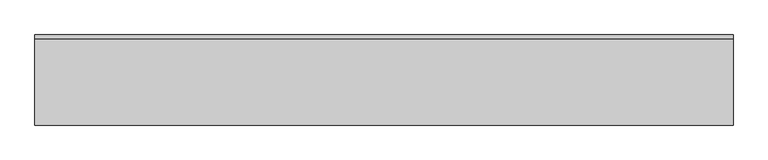
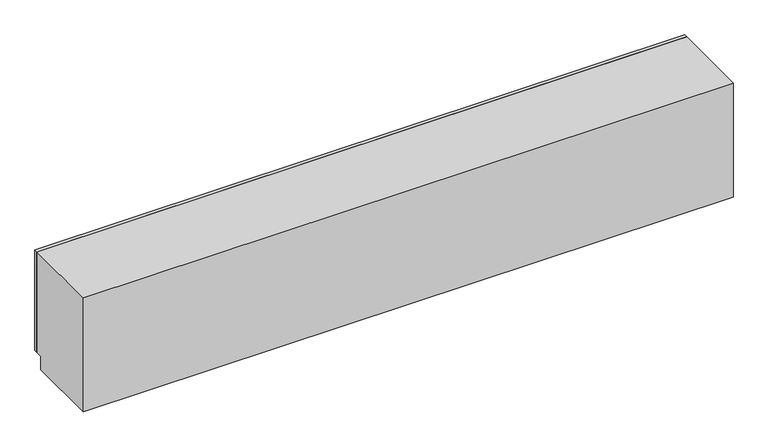
"""IFC4 building model written with IfcOpenShell, lengths in millimetres: furniture geometry, OD_CW_Base Cabinet : OD_CW_Base Cabinet."""

import ifcopenshell
import ifcopenshell.guid

model = None  # the IFC model being written
_history = None  # IfcOwnerHistory: only IFC2X3 demands one
_inside = {}  # id of a spatial element -> (the spatial element, [elements in it])
_under = {}  # id of a project, library or spatial element -> (it, [spatial elements below it])
_declared = {}  # id of a project -> (the project, [libraries it declares])
_typed = {}  # id of a type object -> (the type object, [elements of that type])
_made_of = {}  # id of a material, layer set ... -> (it, [elements and type objects made of it])


def new_model(schema):
    """Start an empty IFC model of exactly this schema.

    Asked for "IFC4X3", IfcOpenShell would pick the latest addendum, in which some entities
    have other attributes; the version numbers below select the first issue.
    IFC2X3 requires an IfcOwnerHistory on every rooted entity: one is made here for all.
    """
    global model, _history
    if schema == "IFC4X3":
        model = ifcopenshell.file(schema_version=(4, 3, 0, 0))
    else:
        model = ifcopenshell.file(schema=schema)
    _inside.clear()
    _under.clear()
    _declared.clear()
    _typed.clear()
    _made_of.clear()
    _history = None
    if model.schema == "IFC2X3":
        org = make("IfcOrganization", Name="unknown")
        user = make(
            "IfcPersonAndOrganization",
            ThePerson=make("IfcPerson", FamilyName="unknown"),
            TheOrganization=org,
        )
        app = make(
            "IfcApplication",
            ApplicationDeveloper=org,
            Version="unknown",
            ApplicationFullName="unknown",
            ApplicationIdentifier="unknown",
        )
        _history = make(
            "IfcOwnerHistory",
            OwningUser=user,
            OwningApplication=app,
            ChangeAction="ADDED",
            CreationDate=0,
        )
    return model


def make(cls, **values):
    """One entity of the class cls with the attributes given. An attribute that is None is left unset."""
    return model.create_entity(
        cls, **{name: value for name, value in values.items() if value is not None}
    )


def rooted(cls, **values):
    """An entity with a GlobalId (a new one), such as an element, a storey or a relation."""
    return make(cls, GlobalId=ifcopenshell.guid.new(), OwnerHistory=_history, **values)


def si_unit(unit_type, name, prefix=None):
    """IfcSIUnit, for example si_unit("LENGTHUNIT", "METRE", prefix="MILLI")."""
    return make("IfcSIUnit", UnitType=unit_type, Prefix=prefix, Name=name)


def assignment(units):
    """IfcUnitAssignment: the units of a project."""
    return None if units is None else make("IfcUnitAssignment", Units=units)


def point(xyz):
    """IfcCartesianPoint."""
    return None if xyz is None else make("IfcCartesianPoint", Coordinates=xyz)


def direction(xyz):
    """IfcDirection."""
    return None if xyz is None else make("IfcDirection", DirectionRatios=xyz)


def frame(location, z_axis=None, x_axis=None):
    """IfcAxis2Placement3D, a coordinate frame: its origin and axes. An axis left out is left unset."""
    return make(
        "IfcAxis2Placement3D",
        Location=point(location),
        Axis=direction(z_axis),
        RefDirection=direction(x_axis),
    )


def origin():
    """The frame at (0, 0, 0) with its axes left unset."""
    return frame((0.0, 0.0, 0.0))


def place(relative_to, where):
    """IfcLocalPlacement: puts the frame where relative to a parent placement (None: the world)."""
    return make(
        "IfcLocalPlacement", PlacementRelTo=relative_to, RelativePlacement=where
    )


def context(
    kind, dimensions, precision=None, world=None, true_north=None, identifier=None
):
    """IfcGeometricRepresentationContext, for example the 3D "Model" context."""
    return make(
        "IfcGeometricRepresentationContext",
        ContextIdentifier=identifier,
        ContextType=kind,
        CoordinateSpaceDimension=dimensions,
        Precision=precision,
        WorldCoordinateSystem=world,
        TrueNorth=true_north,
    )


def project(units=None, contexts=None):
    """IfcProject with its units and contexts."""
    return rooted(
        "IfcProject",
        Name="project",
        RepresentationContexts=contexts,
        UnitsInContext=assignment(units),
    )


def spatial(cls, under=None, at=None, **own):
    """A site, building, storey or space (cls), placed at a placement, below another one or the project."""
    s = rooted(cls, ObjectPlacement=at, **own)
    if under is not None:
        _under.setdefault(under.id(), (under, []))[1].append(s)
    return s


def polyline(points):
    """IfcPolyline through the points."""
    return make("IfcPolyline", Points=[point(p) for p in points])


def outline(outer, holes=None, kind="AREA"):
    """IfcArbitraryClosedProfileDef: a profile drawn as a closed curve; with holes, ...WithVoids."""
    if holes is None:
        return make("IfcArbitraryClosedProfileDef", ProfileType=kind, OuterCurve=outer)
    return make(
        "IfcArbitraryProfileDefWithVoids",
        ProfileType=kind,
        OuterCurve=outer,
        InnerCurves=holes,
    )


def extrude(swept, where, along, depth):
    """IfcExtrudedAreaSolid: the profile swept, set in the frame where, extruded along a direction by depth."""
    return make(
        "IfcExtrudedAreaSolid",
        SweptArea=swept,
        Position=where,
        ExtrudedDirection=direction(along),
        Depth=depth,
    )


def shape(context_of_items, identifier, shape_type, items):
    """IfcShapeRepresentation: the items that make up one representation, for example the "Body"."""
    return make(
        "IfcShapeRepresentation",
        ContextOfItems=context_of_items,
        RepresentationIdentifier=identifier,
        RepresentationType=shape_type,
        Items=items,
    )


def source(mapping_origin, context_of_items, identifier, shape_type, items):
    """IfcRepresentationMap: a shape defined once, which mapped items show again and again."""
    return make(
        "IfcRepresentationMap",
        MappingOrigin=mapping_origin,
        MappedRepresentation=shape(context_of_items, identifier, shape_type, items),
    )


def transform(
    local_origin,
    x_axis=None,
    y_axis=None,
    z_axis=None,
    scale=None,
    scale2=None,
    scale3=None,
    uniform=True,
):
    """IfcCartesianTransformationOperator3D, or its non-uniform kind. x_axis, y_axis, z_axis: its Axis1, 2, 3."""
    if uniform:
        return make(
            "IfcCartesianTransformationOperator3D",
            Axis1=direction(x_axis),
            Axis2=direction(y_axis),
            LocalOrigin=point(local_origin),
            Scale=scale,
            Axis3=direction(z_axis),
        )
    return make(
        "IfcCartesianTransformationOperator3DnonUniform",
        Axis1=direction(x_axis),
        Axis2=direction(y_axis),
        LocalOrigin=point(local_origin),
        Scale=scale,
        Axis3=direction(z_axis),
        Scale2=scale2,
        Scale3=scale3,
    )


def mapped(mapping_source, mapping_target):
    """IfcMappedItem: shows the shape of a source again, moved by a transform."""
    return make(
        "IfcMappedItem", MappingSource=mapping_source, MappingTarget=mapping_target
    )


def made_of(thing, what):
    """Note that an element or type object is made of a material, layer set ...; save() writes the relation."""
    if what is not None:
        _made_of.setdefault(what.id(), (what, []))[1].append(thing)
    return thing


def element(
    cls,
    number,
    at=None,
    inside=None,
    cuts=None,
    type_object=None,
    material=None,
    context=None,
    identifier="Body",
    shape_type=None,
    held_by="IfcProductDefinitionShape",
    body=None,
    shapes=None,
    **own,
):
    """One element of the class cls, such as IfcWall. Its Tag is "e" and its number.

    at: its placement. inside: the storey or other place that contains it. cuts: it is an
    opening in that element (IfcRelVoidsElement). A single representation is given by context,
    identifier, shape_type and body (its items); several are given by shapes. held_by: the class
    of the entity that holds the representations. save() writes the other relations.
    """
    e = rooted(cls, Tag="e%d" % number, ObjectPlacement=at, **own)
    if body is not None:
        shapes = [shape(context, identifier, shape_type, body)]
    if shapes is not None:
        e.Representation = make(held_by, Representations=shapes)
    if inside is not None:
        _inside.setdefault(inside.id(), (inside, []))[1].append(e)
    if cuts is not None:
        rooted(
            "IfcRelVoidsElement", RelatingBuildingElement=cuts, RelatedOpeningElement=e
        )
    if type_object is not None:
        _typed.setdefault(type_object.id(), (type_object, []))[1].append(e)
    return made_of(e, material)


def aggregate(whole, parts):
    """IfcRelAggregates: a whole, such as a stair, and the parts it consists of."""
    return rooted("IfcRelAggregates", RelatingObject=whole, RelatedObjects=parts)


def save(model, path):
    """Write the relations noted so far, then the file.

    IfcRelAggregates (storeys below a building ...), IfcRelContainedInSpatialStructure (elements
    in a storey), IfcRelDefinesByType, IfcRelAssociatesMaterial and IfcRelDeclares: one each for
    every whole, place, type object, material and project.
    """
    for whole, parts in _under.values():
        aggregate(whole, parts)
    for where, things in _inside.values():
        rooted(
            "IfcRelContainedInSpatialStructure",
            RelatedElements=things,
            RelatingStructure=where,
        )
    for kind, things in _typed.values():
        rooted("IfcRelDefinesByType", RelatedObjects=things, RelatingType=kind)
    for what, things in _made_of.values():
        rooted("IfcRelAssociatesMaterial", RelatedObjects=things, RelatingMaterial=what)
    for by, libraries in _declared.values():
        rooted("IfcRelDeclares", RelatingContext=by, RelatedDefinitions=libraries)
    model.write(path)


def furniture_87055c2a(model_context):
    return source(origin(), model_context, "Body", "SweptSolid", [
        extrude(outline(polyline([(18.7377049, -25.4), (18.7377049, 0.0), (4740.5928379, 0.0), (4740.5928379, -25.4), (18.7377049, -25.4)])), frame((0.0, 0.0, 101.6), z_axis=(0.0, 0.0, 1.0), x_axis=(1.0, 0.0, 0.0)), (0.0, 0.0, 1.0), 774.7),
        extrude(outline(polyline([(-25.4, 876.3), (-25.4, 101.6), (-76.2, 101.6), (-76.2, 0.0), (-609.6, 0.0), (-609.6, 876.3), (-25.4, 876.3)])), frame((18.7377049, 0.0, 0.0), z_axis=(1.0, 0.0, 0.0), x_axis=(0.0, 1.0, 0.0)), (0.0, 0.0, 1.0), 4721.855133),
    ])


if __name__ == "__main__":
    model = new_model("IFC4")
    model_context = context("Model", 3, world=origin())
    ifc_project = project(units=[si_unit("LENGTHUNIT", "METRE", prefix="MILLI")], contexts=[model_context])
    site = spatial("IfcSite", under=ifc_project)
    building = spatial("IfcBuilding", under=site)
    placement = place(None, origin())
    furniture_shape = furniture_87055c2a(model_context)
    element("IfcFurniture", 1, ObjectType="OD_CW_Base Cabinet : OD_CW_Base Cabinet", at=placement, inside=building, context=model_context, shape_type="MappedRepresentation", body=[
        mapped(furniture_shape, transform((0.0, 0.0, 0.0), x_axis=(1.0, 0.0, 0.0), y_axis=(0.0, 1.0, 0.0), z_axis=(0.0, 0.0, 1.0))),
    ])
    save(model, "model.ifc")

# Revit data of these elements
# Type "OD_CW_Base Cabinet : OD_CW_Base Cabinet"
#   OD_CW_Width [instance default] = 2' - 10"
#   OD_CW_Length [instance default] = 8' - 0"
#   OD_CW_Height [instance default] = 2' - 3"
#   Depth = 2' - 0"
#   Height = 3' - 0"
#   Width = 4' - 0"
#   OD_CW_Material_Front Panel [instance default] = none
#   OD_CW_Material_Body [instance default] = none
# Element 1 (IfcFurniture, "OD_CW_Base Cabinet : OD_CW_Base Cabinet")
#   OD_CW_Width = 2' - 0"
#   OD_CW_Length = 15' - 5.89981"
#   OD_CW_Height = 2' - 10 1/2"
